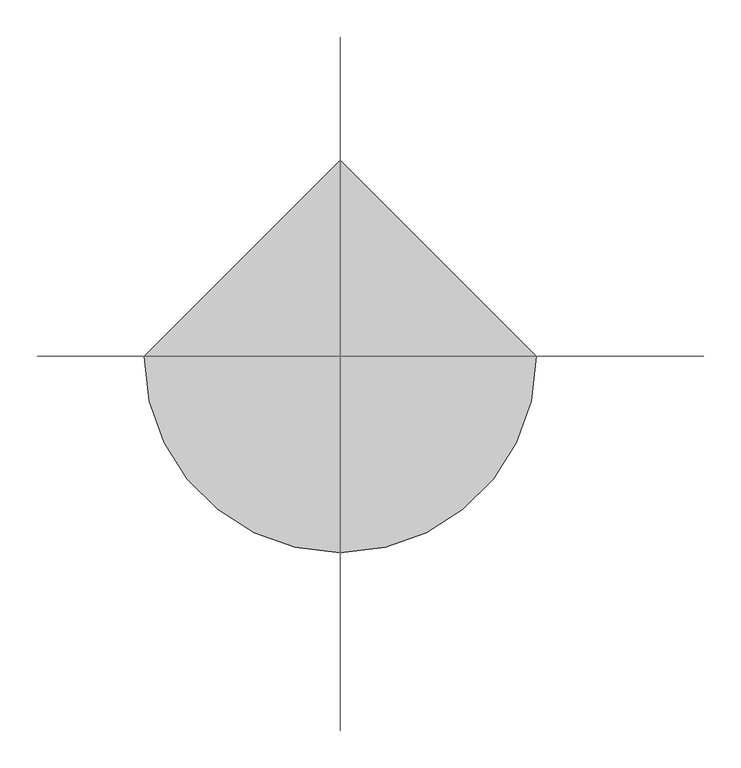
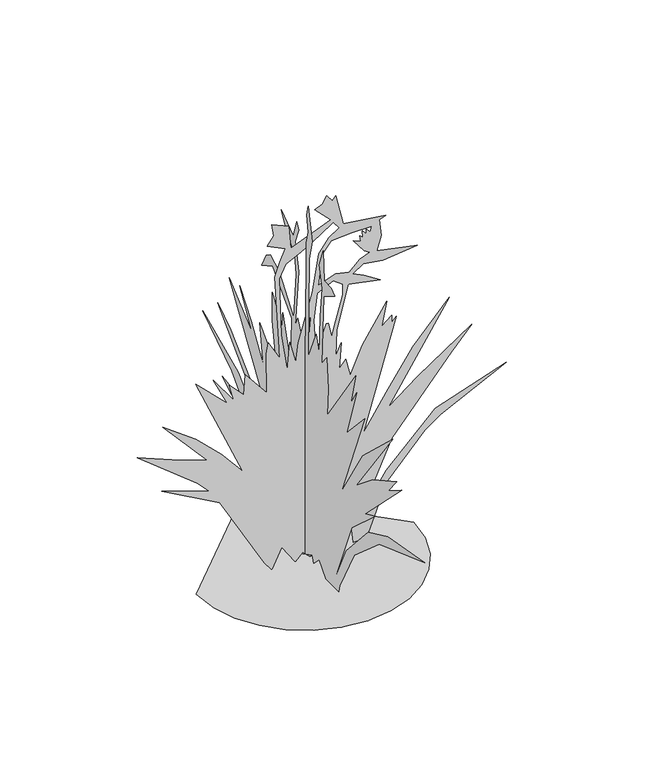
"""IFC4 building model written with IfcOpenShell, lengths in millimetres: proxy geometry, crane lily 26101 : crane lily 26101."""

import ifcopenshell
import ifcopenshell.guid

model = None  # the IFC model being written
_history = None  # IfcOwnerHistory: only IFC2X3 demands one
_inside = {}  # id of a spatial element -> (the spatial element, [elements in it])
_under = {}  # id of a project, library or spatial element -> (it, [spatial elements below it])
_declared = {}  # id of a project -> (the project, [libraries it declares])
_typed = {}  # id of a type object -> (the type object, [elements of that type])
_made_of = {}  # id of a material, layer set ... -> (it, [elements and type objects made of it])


def new_model(schema):
    """Start an empty IFC model of exactly this schema.

    Asked for "IFC4X3", IfcOpenShell would pick the latest addendum, in which some entities
    have other attributes; the version numbers below select the first issue.
    IFC2X3 requires an IfcOwnerHistory on every rooted entity: one is made here for all.
    """
    global model, _history
    if schema == "IFC4X3":
        model = ifcopenshell.file(schema_version=(4, 3, 0, 0))
    else:
        model = ifcopenshell.file(schema=schema)
    _inside.clear()
    _under.clear()
    _declared.clear()
    _typed.clear()
    _made_of.clear()
    _history = None
    if model.schema == "IFC2X3":
        org = make("IfcOrganization", Name="unknown")
        user = make(
            "IfcPersonAndOrganization",
            ThePerson=make("IfcPerson", FamilyName="unknown"),
            TheOrganization=org,
        )
        app = make(
            "IfcApplication",
            ApplicationDeveloper=org,
            Version="unknown",
            ApplicationFullName="unknown",
            ApplicationIdentifier="unknown",
        )
        _history = make(
            "IfcOwnerHistory",
            OwningUser=user,
            OwningApplication=app,
            ChangeAction="ADDED",
            CreationDate=0,
        )
    return model


def make(cls, **values):
    """One entity of the class cls with the attributes given. An attribute that is None is left unset."""
    return model.create_entity(
        cls, **{name: value for name, value in values.items() if value is not None}
    )


def rooted(cls, **values):
    """An entity with a GlobalId (a new one), such as an element, a storey or a relation."""
    return make(cls, GlobalId=ifcopenshell.guid.new(), OwnerHistory=_history, **values)


def si_unit(unit_type, name, prefix=None):
    """IfcSIUnit, for example si_unit("LENGTHUNIT", "METRE", prefix="MILLI")."""
    return make("IfcSIUnit", UnitType=unit_type, Prefix=prefix, Name=name)


def assignment(units):
    """IfcUnitAssignment: the units of a project."""
    return None if units is None else make("IfcUnitAssignment", Units=units)


def point(xyz):
    """IfcCartesianPoint."""
    return None if xyz is None else make("IfcCartesianPoint", Coordinates=xyz)


def direction(xyz):
    """IfcDirection."""
    return None if xyz is None else make("IfcDirection", DirectionRatios=xyz)


def frame(location, z_axis=None, x_axis=None):
    """IfcAxis2Placement3D, a coordinate frame: its origin and axes. An axis left out is left unset."""
    return make(
        "IfcAxis2Placement3D",
        Location=point(location),
        Axis=direction(z_axis),
        RefDirection=direction(x_axis),
    )


def origin():
    """The frame at (0, 0, 0) with its axes left unset."""
    return frame((0.0, 0.0, 0.0))


def place(relative_to, where):
    """IfcLocalPlacement: puts the frame where relative to a parent placement (None: the world)."""
    return make(
        "IfcLocalPlacement", PlacementRelTo=relative_to, RelativePlacement=where
    )


def context(
    kind, dimensions, precision=None, world=None, true_north=None, identifier=None
):
    """IfcGeometricRepresentationContext, for example the 3D "Model" context."""
    return make(
        "IfcGeometricRepresentationContext",
        ContextIdentifier=identifier,
        ContextType=kind,
        CoordinateSpaceDimension=dimensions,
        Precision=precision,
        WorldCoordinateSystem=world,
        TrueNorth=true_north,
    )


def project(units=None, contexts=None):
    """IfcProject with its units and contexts."""
    return rooted(
        "IfcProject",
        Name="project",
        RepresentationContexts=contexts,
        UnitsInContext=assignment(units),
    )


def spatial(cls, under=None, at=None, **own):
    """A site, building, storey or space (cls), placed at a placement, below another one or the project."""
    s = rooted(cls, ObjectPlacement=at, **own)
    if under is not None:
        _under.setdefault(under.id(), (under, []))[1].append(s)
    return s


def point_list(points):
    """IfcCartesianPointList2D or 3D."""
    cls = (
        "IfcCartesianPointList2D" if len(points[0]) == 2 else "IfcCartesianPointList3D"
    )
    return make(cls, CoordList=points)


def triangles(points, corners, closed=None, point_numbers=None):
    """IfcTriangulatedFaceSet: each triangle names its three corners, points numbered from 1."""
    return make(
        "IfcTriangulatedFaceSet",
        Coordinates=point_list(points),
        Closed=closed,
        CoordIndex=corners,
        PnIndex=point_numbers,
    )


def shape(context_of_items, identifier, shape_type, items):
    """IfcShapeRepresentation: the items that make up one representation, for example the "Body"."""
    return make(
        "IfcShapeRepresentation",
        ContextOfItems=context_of_items,
        RepresentationIdentifier=identifier,
        RepresentationType=shape_type,
        Items=items,
    )


def source(mapping_origin, context_of_items, identifier, shape_type, items):
    """IfcRepresentationMap: a shape defined once, which mapped items show again and again."""
    return make(
        "IfcRepresentationMap",
        MappingOrigin=mapping_origin,
        MappedRepresentation=shape(context_of_items, identifier, shape_type, items),
    )


def transform(
    local_origin,
    x_axis=None,
    y_axis=None,
    z_axis=None,
    scale=None,
    scale2=None,
    scale3=None,
    uniform=True,
):
    """IfcCartesianTransformationOperator3D, or its non-uniform kind. x_axis, y_axis, z_axis: its Axis1, 2, 3."""
    if uniform:
        return make(
            "IfcCartesianTransformationOperator3D",
            Axis1=direction(x_axis),
            Axis2=direction(y_axis),
            LocalOrigin=point(local_origin),
            Scale=scale,
            Axis3=direction(z_axis),
        )
    return make(
        "IfcCartesianTransformationOperator3DnonUniform",
        Axis1=direction(x_axis),
        Axis2=direction(y_axis),
        LocalOrigin=point(local_origin),
        Scale=scale,
        Axis3=direction(z_axis),
        Scale2=scale2,
        Scale3=scale3,
    )


def mapped(mapping_source, mapping_target):
    """IfcMappedItem: shows the shape of a source again, moved by a transform."""
    return make(
        "IfcMappedItem", MappingSource=mapping_source, MappingTarget=mapping_target
    )


def made_of(thing, what):
    """Note that an element or type object is made of a material, layer set ...; save() writes the relation."""
    if what is not None:
        _made_of.setdefault(what.id(), (what, []))[1].append(thing)
    return thing


def element(
    cls,
    number,
    at=None,
    inside=None,
    cuts=None,
    type_object=None,
    material=None,
    context=None,
    identifier="Body",
    shape_type=None,
    held_by="IfcProductDefinitionShape",
    body=None,
    shapes=None,
    **own,
):
    """One element of the class cls, such as IfcWall. Its Tag is "e" and its number.

    at: its placement. inside: the storey or other place that contains it. cuts: it is an
    opening in that element (IfcRelVoidsElement). A single representation is given by context,
    identifier, shape_type and body (its items); several are given by shapes. held_by: the class
    of the entity that holds the representations. save() writes the other relations.
    """
    e = rooted(cls, Tag="e%d" % number, ObjectPlacement=at, **own)
    if body is not None:
        shapes = [shape(context, identifier, shape_type, body)]
    if shapes is not None:
        e.Representation = make(held_by, Representations=shapes)
    if inside is not None:
        _inside.setdefault(inside.id(), (inside, []))[1].append(e)
    if cuts is not None:
        rooted(
            "IfcRelVoidsElement", RelatingBuildingElement=cuts, RelatedOpeningElement=e
        )
    if type_object is not None:
        _typed.setdefault(type_object.id(), (type_object, []))[1].append(e)
    return made_of(e, material)


def aggregate(whole, parts):
    """IfcRelAggregates: a whole, such as a stair, and the parts it consists of."""
    return rooted("IfcRelAggregates", RelatingObject=whole, RelatedObjects=parts)


def save(model, path):
    """Write the relations noted so far, then the file.

    IfcRelAggregates (storeys below a building ...), IfcRelContainedInSpatialStructure (elements
    in a storey), IfcRelDefinesByType, IfcRelAssociatesMaterial and IfcRelDeclares: one each for
    every whole, place, type object, material and project.
    """
    for whole, parts in _under.values():
        aggregate(whole, parts)
    for where, things in _inside.values():
        rooted(
            "IfcRelContainedInSpatialStructure",
            RelatedElements=things,
            RelatingStructure=where,
        )
    for kind, things in _typed.values():
        rooted("IfcRelDefinesByType", RelatedObjects=things, RelatingType=kind)
    for what, things in _made_of.values():
        rooted("IfcRelAssociatesMaterial", RelatedObjects=things, RelatingMaterial=what)
    for by, libraries in _declared.values():
        rooted("IfcRelDeclares", RelatingContext=by, RelatedDefinitions=libraries)
    model.write(path)


def entourage_55f6ff97(model_context):
    return source(origin(), model_context, "Body", "Tessellation", [
        triangles([(-264.3380075, 0.0, 0.0272524), (-257.3504617, -60.5688865, 0.0272524), (-237.4475159, -116.1916269, 0.0272524), (-206.2245489, -165.274632, 0.0272524), (-165.274632, -206.2245489, 0.0272524), (-116.1916269, -237.4475159, 0.0272524), (-60.5688865, -257.3504617, 0.0272524), (1.16e-05, -264.3380075, 0.0272524), (60.5688865, -257.3504617, 0.0272524), (116.1916269, -237.4475159, 0.0272524), (165.274632, -206.2245489, 0.0272524), (206.2245489, -165.274632, 0.0272524), (237.4475159, -116.1916269, 0.0272524), (257.3504617, -60.5688865, 0.0272524), (264.3380075, 2.31e-05, 0.0272524), (-3.47e-05, 264.3380075, 0.0272524), (-5.2e-06, -141.3706678, 0.0), (-2.8e-06, -89.4159448, 0.054498), (-3.14e-05, -59.9343958, 33.2735186), (-3.1e-05, -36.3827356, 9.846953), (-3.03e-05, -30.3380374, 26.1345898), (2.2e-06, 22.1351019, 0.0353721), (-2.75e-05, 35.0893666, 22.475361), (-2.7e-05, 50.4325003, 13.9824575), (-2.41e-05, 71.8028075, 80.7852761), (5.2e-06, 91.613049, 0.0211753), (-2.36e-05, 109.0153662, 40.8424698), (-2.42e-05, 112.8357816, 15.9965016), (-1.83e-05, 164.4437961, 134.5614359), (-1.5e-05, 201.3025201, 190.8125718), (-8.6e-06, 314.8967674, 236.0083596), (-6.4e-06, 348.2342674, 257.8737037), (-8.8e-06, 301.5160253, 250.5209003), (-1.18e-05, 246.732487, 231.9590791), (-7.1e-06, 309.0598417, 295.0364789), (8e-07, 430.3017509, 376.6543714), (-7.9e-06, 280.4721063, 309.3519387), (-1.58e-05, 174.5674878, 204.3200503), (-9.8e-06, 240.1660818, 307.4037292), (-3e-07, 367.670363, 434.9626582), (-3.8e-06, 312.5929836, 399.2629114), (-1.14e-05, 210.1351387, 300.3374635), (-1.65e-05, 148.1844779, 220.8381918), (-1.17e-05, 187.1702069, 323.3016323), (3e-07, 320.1596366, 527.8276657), (-6.4e-06, 222.976615, 445.7627257), (-1.5e-06, 274.807899, 534.3072121), (-5.5e-06, 226.7299833, 472.9153562), (-1.02e-05, 175.4651256, 391.7724529), (-6.5e-06, 190.5821898, 491.1144633), (-1.2e-05, 119.3145649, 415.5265626), (-7.8e-06, 137.4532288, 529.6031387), (-5.6e-06, 138.7511692, 601.2540341), (-9.5e-06, 94.9513718, 536.1969586), (-8.4e-06, 93.3989229, 575.3383922), (-1.32e-05, 59.5732078, 463.4487828), (-9.8e-06, 56.2066891, 583.9388483), (-3.7e-06, 136.0049161, 669.1432405), (-2.4e-06, 181.9436545, 644.4467829), (-2.1e-06, 163.9243692, 680.6875214), (-2.5e-06, 147.0399529, 691.5511024), (-4.8e-06, 108.1804607, 671.9067347), (-1e-05, 48.046931, 590.4565101), (-6.9e-06, 36.8709235, 709.0745968), (-5.3e-06, 43.8627887, 753.7100264), (-2e-06, 83.7514831, 804.4440662), (-3e-07, 99.8779606, 836.6538008), (-3.7e-06, 49.136086, 799.8898384), (-2.9e-06, 35.0893666, 845.2923723), (-3.8e-06, 26.4505657, 828.0152292), (-4.3e-06, 41.5678933, 791.3020632), (-7e-06, 26.8495989, 721.233593), (-1.07e-05, 41.5678933, 575.3383922), (-1.05e-05, 30.7698379, 599.0950453), (-1.29e-05, 9.1735731, 551.5843188), (-1.27e-05, -4.2437592, 577.167205), (-5.7e-06, -6.2811965, 815.731822), (-5.1e-06, -13.569935, 847.4513248), (-3.6e-06, -6.9461944, 887.7586756), (-3.1e-06, -14.582304, 914.4007267), (-6.2e-06, -30.3001922, 833.2324253), (-7.2e-06, -17.1413308, 780.7407166), (-1.46e-05, -14.582304, 527.8276657), (-1.38e-05, -46.9765748, 605.5745916), (-1.57e-05, -59.9343958, 560.222854), (-1.28e-05, -63.7807226, 662.0591526), (-1.1e-05, -73.6229771, 738.5157503), (-8.8e-06, -59.9343958, 791.3020632), (-8.5e-06, -68.5729447, 815.05868), (-8.2e-06, -77.2114935, 838.812826), (-1.06e-05, -81.5307611, 763.227396), (-1.2e-05, -110.9300204, 761.8202871), (-1.3e-05, -126.4778813, 751.5510738), (-1.23e-05, -100.3333834, 735.2899298), (-1.17e-05, -79.708316, 722.0590513), (-1.66e-05, -70.7324513, 545.1047725), (-1.68e-05, -92.3897821, 572.3361045), (-1.94e-05, -98.8076044, 495.4324774), (-2.12e-05, -94.4883277, 426.3240867), (-2.14e-05, -213.2677237, 599.0950453), (-2.3e-05, -193.8311193, 517.0301053), (-2.28e-05, -217.5869913, 558.0613217), (-2.48e-05, -176.5542669, 430.6446442), (-2.57e-05, -252.1411685, 512.7095841), (-2.87e-05, -152.798395, 264.3532501), (-2.83e-05, -244.4081376, 413.0424482), (-3.04e-05, -369.3264393, 531.0712541), (-2.98e-05, -215.4274755, 318.343541), (-3.13e-05, -285.475907, 376.1107999), (-3.42e-05, -387.58906, 431.8587779), (-3.39e-05, -351.4829427, 387.4518954), (-3.53e-05, -406.9616784, 422.1127885), (-3.3e-05, -254.1018046, 269.3443517), (-3.43e-05, -295.3336628, 288.109885), (-3.26e-05, -197.6014924, 198.8161167), (-3.48e-05, -118.2442087, 7.3579794), (-3.37e-05, -173.2017281, 125.4509545), (-3.48e-05, -266.8272088, 229.6761334), (-3.73e-05, -347.9879162, 267.302198), (-4.35e-05, -504.8177693, 294.5894314), (-3.69e-05, -312.1281501, 226.3418711), (-3.5e-05, -207.3218293, 133.5593986), (-3.57e-05, -146.3193573, 18.1561127), (117.3305654, 2.31e-05, 0.0405123), (110.3389591, 2.08e-05, 74.4091073), (78.0842327, 2.54e-05, 21.0145808), (55.6151237, 2.49e-05, 46.2313396), (12.5873108, 2.89e-05, 0.0122306), (-5.1707583, 2.92e-05, 18.1490262), (-24.1045425, 3.09e-05, 0.0037426), (-56.6857342, 2.97e-05, 48.3908508), (-81.2114855, 3.28e-05, 0.0181663), (-98.986418, 3.3e-05, 24.1438615), (-207.7917316, 2.63e-05, 216.6390658), (-348.2342674, 2.78e-05, 294.5894314), (-233.774666, 2.51e-05, 255.7146967), (-261.6024369, 2.45e-05, 285.2828592), (-408.7041229, 2.4e-05, 402.5700133), (-324.6782925, 2.24e-05, 368.0386909), (-238.0939517, 2.05e-05, 335.6206115), (-346.0752786, 1.79e-05, 458.719275), (-266.2303157, 1.79e-05, 400.2179767), (-203.8244956, 1.88e-05, 339.715129), (-151.7089902, 2.02e-05, 277.3123428), (-266.1693456, 9.5e-06, 540.784215), (-189.3886398, 1.06e-05, 466.0141786), (-222.976615, 7.9e-06, 536.4662009), (-173.7341084, 9.8e-06, 467.1774796), (-184.1031521, 7.7e-06, 510.5505589), (-149.5492202, 8.4e-06, 473.8373929), (-145.2299525, 5.2e-06, 523.5096517), (-93.3989229, 6.8e-06, 458.719275), (-94.0984351, 9e-07, 559.4354384), (-89.0799006, -9e-07, 586.138496), (-61.0044976, 8e-07, 536.4662009), (-64.4230889, -1.9e-06, 583.7153154), (-73.364658, -1.14e-05, 749.2980864), (-61.7167134, -1.39e-05, 783.3111992), (-47.9079951, -1.63e-05, 813.4864649), (-91.2394163, -1.57e-05, 834.4947756), (-76.5455003, -1.76e-05, 856.3946743), (-80.4413563, -1.92e-05, 886.3260595), (-39.8899707, -2e-05, 869.0464457), (-35.0893666, -1.67e-05, 810.7381588), (62.093907, -2.33e-05, 849.6128935), (23.2207756, -2.39e-05, 888.4850847), (42.4165107, -2.52e-05, 896.5013105), (53.4556125, -2.67e-05, 914.4007267), (66.1944834, -2.63e-05, 896.8848627), (74.7598808, -2.72e-05, 906.7806976), (93.6785752, -2.34e-05, 828.1498867), (196.1872255, -2.7e-05, 813.9157265), (180.8732984, -2.6e-05, 808.5791336), (185.7325766, -2.37e-05, 766.8723043), (174.394515, -2.11e-05, 730.8322803), (273.7385602, -2.41e-05, 709.2371595), (189.3833167, -2e-05, 700.9592491), (142.0676456, -1.83e-05, 708.1576469), (116.0844387, -1.62e-05, 691.9600891), (142.8525086, -1.66e-05, 679.102589), (183.0330503, -1.68e-05, 653.0853544), (105.3178811, -1.44e-05, 669.0848139), (77.0491851, -6.7e-06, 560.5047772), (75.051728, -2.7e-06, 495.4324774), (87.9216592, -5e-06, 524.393573), (83.6900225, -9e-07, 458.719275), (98.8076044, -2.7e-06, 478.1553706), (109.6056554, -5e-07, 432.803633), (138.9439536, -5.8e-06, 499.7708027), (199.0078928, -1.39e-05, 592.0084502), (187.352336, -9.8e-06, 532.1482232), (211.1082079, -1.2e-05, 551.5843188), (211.1082079, -1.1e-05, 534.3072121), (221.9062589, -1.21e-05, 545.1047725), (142.0000807, 7.6e-06, 272.9918035), (197.3987977, 1e-07, 358.912431), (262.4025334, -8.4e-06, 452.8214155), (351.4829427, -1.8e-05, 549.4227502), (202.4694002, 2.3e-06, 318.343541), (273.8909673, -4.1e-06, 372.7275035), (405.4757589, -1.51e-05, 460.8783002), (355.6612487, -9.6e-06, 405.7856601), (211.5270596, 6.8e-06, 235.3906284), (131.6828507, 2.08e-05, 59.5396797), (197.4798247, 1.2e-05, 158.3333043), (317.0659301, -2e-07, 275.0161712), (489.6996878, -1.12e-05, 333.4616226), (330.1571005, 5e-07, 255.2422691), (291.8284444, 3.8e-06, 227.7759587), (199.2240496, 1.38e-05, 127.0808696), (148.478864, 2.13e-05, 0.0507429), (114.3788288, -2.24e-05, 797.4488537), (63.6714996, -2.01e-05, 794.7361559), (42.3199913, -1.75e-05, 767.5631779), (31.8592449, -1.25e-05, 691.9600891), (74.6966352, -1.53e-05, 706.3237473), (107.4461487, -1.62e-05, 698.437092), (132.807564, -1.88e-05, 722.7067589), (157.1176626, -2.05e-05, 732.9912329), (143.9299774, -2.04e-05, 741.276701), (117.5705943, -2.13e-05, 776.2906248), (135.9680906, -2.16e-05, 768.3049204), (133.7021497, -2.24e-05, 783.2401279), (140.693002, -2.24e-05, 777.0983517), (139.840574, -2.33e-05, 793.4610884), (148.478864, -2.3e-05, 782.6634916), (148.8047525, -2.38e-05, 795.162874), (158.4753014, -2.36e-05, 785.4854851), (162.2614257, -2.45e-05, 797.6698431), (36.4967821, -2.03e-05, 819.0008085), (-10.5179706, -1.66e-05, 790.7762959), (-46.6034508, -1.4e-05, 773.6338102), (-62.8378705, -1.14e-05, 741.9143074), (-57.6440741, -2.8e-06, 594.8100597), (-43.7276589, 2.2e-06, 499.7530349), (-37.2488755, -2.2e-06, 568.8613893), (-22.1313685, 5e-07, 512.7095841), (-15.8925131, -2.6e-06, 559.8647), (18.0916476, -1.1e-05, 677.0451565), (33.6138798, -1.74e-05, 772.2038103), (57.6697312, -2.04e-05, 805.3914648), (83.6900225, -2.25e-05, 821.5356829), (68.5729447, -2.3e-05, 840.9743219), (30.2087529, -1.13e-05, 671.65784), (21.8014718, -6.9e-06, 605.0462809), (25.6817059, -2.5e-06, 528.0867342), (30.8554363, -2.8e-06, 528.7344418), (51.5501011, -7.1e-06, 586.290885), (56.0771503, -7.3e-06, 585.6457209), (65.1309854, -5.4e-06, 548.1349654), (69.6580301, -6.8e-06, 568.1831966), (91.6460685, -1.24e-05, 645.7879074), (91.6460685, -1.4e-05, 672.9507116), (68.3644091, -1.4e-05, 690.4106197), (6.9271952, -5.7e-06, 595.3460009), (10.8074288, -4.5e-06, 573.3571904), (13.394269, -6.1e-06, 597.9317079), (15.3343985, -7.9e-06, 627.035055)], [[15, 16, 1], [14, 15, 1], [14, 1, 2], [13, 14, 2], [13, 2, 3], [13, 3, 4], [12, 13, 4], [11, 12, 4], [11, 4, 5], [11, 5, 6], [11, 6, 7], [11, 7, 8], [11, 8, 9], [11, 9, 10], [46, 47, 48], [119, 120, 121], [35, 36, 37], [106, 107, 108], [39, 40, 41], [39, 41, 42], [101, 102, 103], [111, 112, 113], [105, 106, 108], [44, 45, 46], [113, 114, 115], [54, 55, 56], [103, 104, 105], [99, 100, 101], [109, 110, 111], [89, 90, 91], [118, 119, 121], [31, 32, 33], [46, 48, 49], [44, 46, 49], [79, 80, 81], [78, 79, 81], [66, 67, 68], [27, 28, 29], [52, 53, 54], [88, 89, 91], [87, 88, 91], [49, 50, 51], [58, 59, 60], [99, 101, 103], [25, 26, 27], [83, 84, 85], [109, 111, 113], [108, 109, 113], [96, 97, 98], [68, 69, 70], [68, 70, 71], [38, 39, 42], [38, 42, 43], [65, 66, 68], [65, 68, 71], [65, 71, 72], [64, 65, 72], [64, 72, 73], [63, 64, 73], [118, 121, 122], [117, 118, 122], [117, 122, 123], [116, 117, 123], [73, 74, 75], [116, 123, 17], [116, 17, 18], [58, 60, 61], [58, 61, 62], [57, 58, 62], [57, 62, 63], [77, 78, 81], [77, 81, 82], [76, 77, 82], [76, 82, 83], [75, 76, 83], [92, 93, 94], [19, 20, 21], [30, 31, 33], [30, 33, 34], [91, 92, 94], [87, 91, 94], [87, 94, 95], [86, 87, 95], [86, 95, 96], [85, 86, 96], [34, 35, 37], [34, 37, 38], [30, 34, 38], [25, 27, 29], [57, 63, 73], [56, 57, 73], [56, 73, 75], [56, 75, 83], [23, 24, 25], [99, 103, 105], [29, 30, 38], [105, 108, 113], [105, 113, 115], [51, 52, 54], [51, 54, 56], [83, 85, 96], [21, 22, 23], [83, 96, 98], [83, 98, 99], [56, 83, 99], [29, 38, 43], [25, 29, 43], [115, 116, 18], [115, 18, 19], [105, 115, 19], [21, 23, 25], [44, 49, 51], [43, 44, 51], [56, 99, 105], [51, 56, 105], [43, 51, 105], [43, 105, 19], [25, 43, 19], [21, 25, 19], [248, 124, 125], [241, 229, 212], [206, 207, 208], [197, 198, 199], [146, 147, 148], [134, 135, 136], [196, 197, 199], [241, 212, 213], [255, 237, 238], [140, 141, 142], [200, 201, 202], [137, 138, 139], [255, 238, 239], [258, 255, 239], [175, 176, 177], [184, 185, 186], [235, 236, 237], [180, 181, 182], [189, 190, 191], [144, 145, 146], [140, 142, 143], [247, 248, 125], [171, 172, 173], [200, 202, 203], [199, 200, 203], [193, 194, 195], [237, 255, 256], [220, 221, 222], [148, 149, 150], [137, 139, 140], [224, 225, 226], [229, 241, 242], [195, 196, 199], [222, 223, 224], [153, 154, 155], [179, 180, 182], [150, 151, 152], [226, 227, 228], [191, 192, 193], [186, 187, 188], [169, 170, 171], [175, 177, 178], [152, 153, 155], [195, 199, 203], [161, 162, 163], [240, 241, 213], [240, 213, 214], [165, 166, 167], [167, 168, 169], [165, 167, 169], [165, 169, 171], [191, 193, 195], [189, 191, 195], [188, 189, 195], [239, 240, 214], [239, 214, 215], [125, 126, 127], [124, 248, 249], [124, 249, 250], [161, 163, 164], [160, 161, 164], [159, 160, 164], [131, 132, 133], [144, 146, 148], [129, 130, 131], [131, 133, 134], [206, 208, 209], [205, 206, 209], [205, 209, 210], [204, 205, 210], [204, 210, 211], [204, 211, 124], [204, 124, 250], [246, 247, 125], [195, 203, 204], [144, 148, 150], [144, 150, 152], [158, 159, 164], [127, 128, 129], [246, 125, 127], [246, 127, 129], [246, 129, 131], [136, 137, 140], [136, 140, 143], [136, 143, 144], [134, 136, 144], [131, 134, 144], [220, 222, 224], [220, 224, 226], [220, 226, 228], [219, 220, 228], [131, 144, 152], [258, 239, 215], [174, 175, 178], [186, 188, 195], [215, 216, 217], [131, 152, 155], [157, 158, 164], [217, 218, 219], [186, 195, 204], [219, 228, 229], [245, 246, 131], [245, 131, 215], [244, 245, 215], [254, 244, 215], [254, 215, 217], [253, 254, 217], [252, 253, 217], [257, 258, 215], [184, 186, 204], [184, 204, 250], [183, 184, 250], [183, 250, 251], [182, 183, 251], [182, 251, 252], [182, 252, 217], [179, 182, 217], [179, 217, 219], [178, 179, 219], [174, 178, 219], [174, 219, 229], [173, 174, 229], [171, 173, 229], [171, 229, 242], [165, 171, 242], [165, 242, 243], [165, 243, 230], [164, 165, 230], [164, 230, 231], [164, 231, 232], [157, 164, 232], [157, 232, 233], [156, 157, 233], [156, 233, 234], [156, 234, 235], [155, 156, 235], [131, 155, 235], [131, 235, 237], [131, 237, 256], [215, 131, 256], [257, 215, 256]], closed=False),
    ])


if __name__ == "__main__":
    model = new_model("IFC4")
    model_context = context("Model", 3, world=origin())
    ifc_project = project(units=[si_unit("LENGTHUNIT", "METRE", prefix="MILLI")], contexts=[model_context])
    site = spatial("IfcSite", under=ifc_project)
    building = spatial("IfcBuilding", under=site)
    placement = place(None, origin())
    entourage_shape = entourage_55f6ff97(model_context)
    element("IfcBuildingElementProxy", 1, Name="crane lily 26101 : crane lily 26101", ObjectType="crane lily 26101 : crane lily 26101", at=placement, inside=building, context=model_context, shape_type="MappedRepresentation", body=[
        mapped(entourage_shape, transform((0.0, 0.0, 0.0), x_axis=(1.0, 0.0, 0.0), y_axis=(0.0, 1.0, 0.0), z_axis=(0.0, 0.0, 1.0))),
    ])
    save(model, "model.ifc")

# Revit data of these elements
# Type "crane lily 26101 : crane lily 26101"
#   built-in parameter 1005195 = "RPC-16-FWM5-GM7X-C67P-4000-ST1L-LVER-AU"
#   Height = 0
